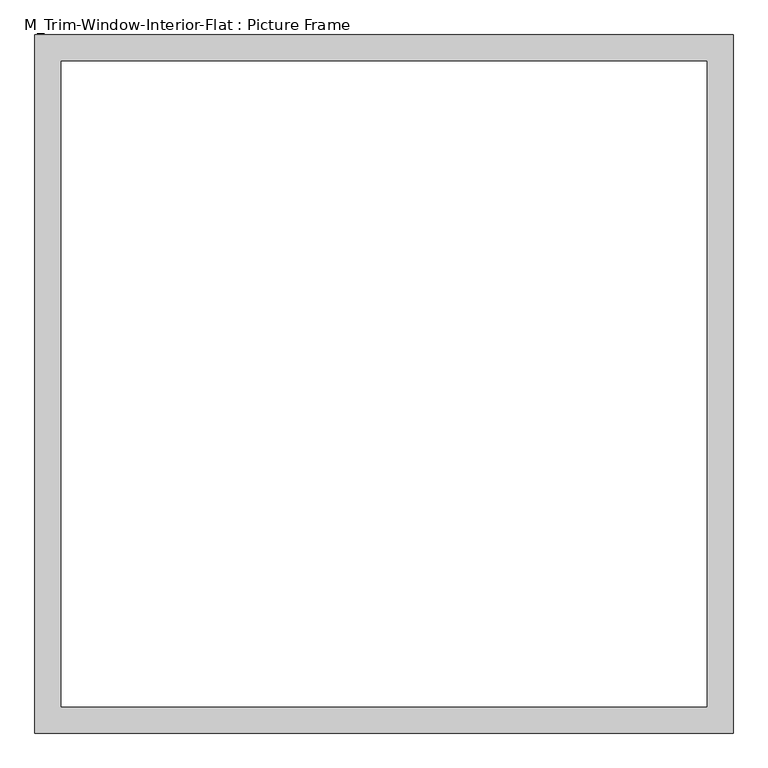
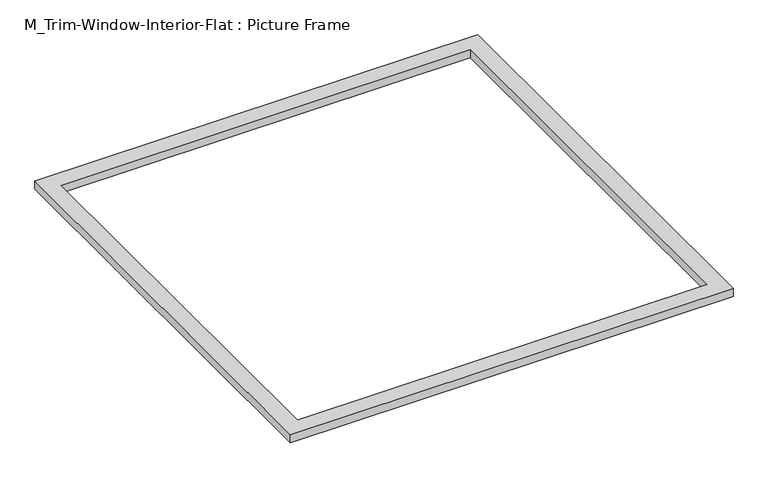
"""IFC4 building model written with IfcOpenShell, lengths in millimetres: proxy geometry, M_Trim-Window-Interior-Flat : Picture Frame."""

from ifc_helpers import new_model, si_unit, origin, origin_with_axes, place, context, project, spatial, polyline, outline, extrude, source, transform, mapped, element, save


def m_trim_window_interior_flat_picture_frame_2e224720(model_context):
    return source(origin(), model_context, "Body", "SweptSolid", [
        extrude(outline(polyline([(797.3, 47.3), (797.3, -1547.3), (-797.3, -1547.3), (-797.3, 47.3), (797.3, 47.3)]), holes=[polyline([(737.3, -12.7), (-737.3, -12.7), (-737.3, -1487.3), (737.3, -1487.3), (737.3, -12.7)])]), origin_with_axes(), (0.0, 0.0, 1.0), 30.0),
    ])


if __name__ == "__main__":
    model = new_model("IFC4")
    model_context = context("Model", 3, world=origin())
    ifc_project = project(units=[si_unit("LENGTHUNIT", "METRE", prefix="MILLI")], contexts=[model_context])
    site = spatial("IfcSite", under=ifc_project)
    building = spatial("IfcBuilding", under=site)
    placement = place(None, origin())
    m_trim_window_interior_flat_picture_frame_shape = m_trim_window_interior_flat_picture_frame_2e224720(model_context)
    element("IfcBuildingElementProxy", 1, Name="M_Trim-Window-Interior-Flat : Picture Frame", ObjectType="M_Trim-Window-Interior-Flat : Picture Frame", at=placement, inside=building, context=model_context, shape_type="MappedRepresentation", body=[
        mapped(m_trim_window_interior_flat_picture_frame_shape, transform((0.0, 0.0, 0.0), x_axis=(1.0, 0.0, 0.0), y_axis=(0.0, 1.0, 0.0), z_axis=(0.0, 0.0, 1.0))),
    ])
    save(model, "model.ifc")

# Revit data of these elements
# Type "M_Trim-Window-Interior-Flat : Picture Frame"
#   Trim Thickness_Picture Frame = 0.03 m
#   Trim Width = 0.06 m
#   Trim Thickness_with Sill = 0.02 m
#   Sill Thickness = 0.03 m
#   Opening Width [instance default] = 0.6 m
#   Opening Height [instance default] = 0.9 m
#   Default Elevation = 1.2 m
#   Sill = no
#   Picture Frame = yes
#   Trim Material [instance default] = none
# Element 1 (IfcBuildingElementProxy, "M_Trim-Window-Interior-Flat : Picture Frame")
#   Opening Width = 1.5 m
#   Opening Height = 1.5 m
#   Trim Material = Wood - Stained
#   Materials on its faces: "Wood - Stained"
# Materials
#   "Wood - Stained": class "Wood", colour RGB 224 178 126, transparency 0, Cost = 0
